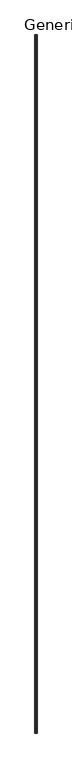
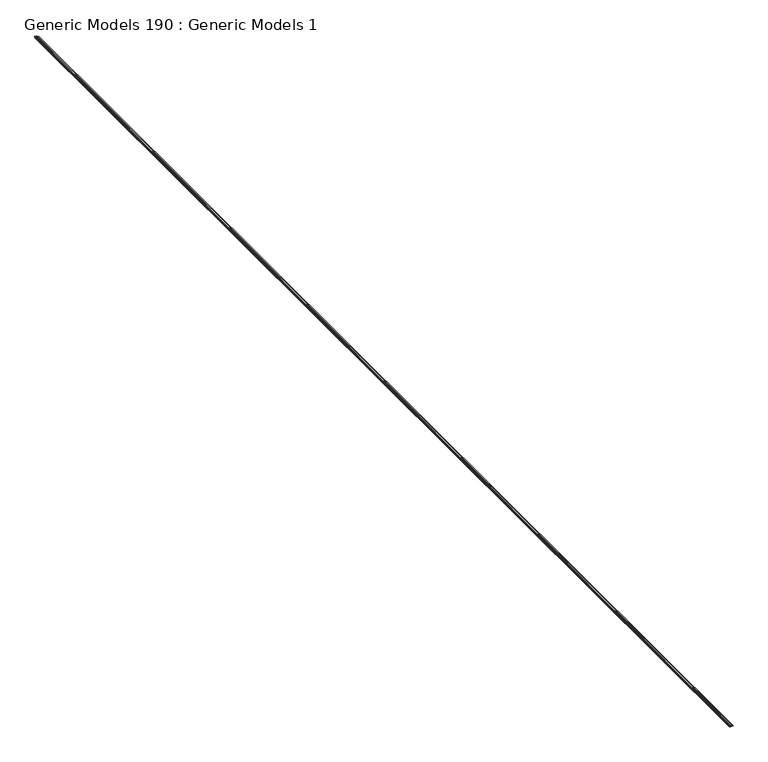
"""IFC4 building model written with IfcOpenShell, lengths in millimetres: proxy geometry, Generic Models 190 : Generic Models 1."""

from ifc_helpers import new_model, si_unit, frame, origin, place, context, project, spatial, polyline, outline, extrude, source, transform, mapped, element, save


def generic_models_190_generic_models_1_2642ba55(model_context):
    return source(origin(), model_context, "Body", "SweptSolid", [
        extrude(outline(polyline([(142599.5579199, -6986.3995748), (142601.7677199, -6986.3995748), (142601.7677199, -6985.5407339), (142622.0822986, -6985.5407339), (142622.0822986, -6986.8107339), (142603.0377199, -6986.8107339), (142603.0377199, -6987.6695748), (142598.2879199, -6987.6695748), (142598.2879199, -6965.4445748), (142609.7179199, -6965.4445748), (142609.7179199, -6952.7445748), (142598.2879199, -6952.7445748), (142598.2879199, -6929.0313908), (142599.5579199, -6929.0313908), (142599.5579199, -6951.4745748), (142610.9879199, -6951.4745748), (142610.9879199, -6966.7145748), (142599.5579199, -6966.7145748), (142599.5579199, -6986.3995748)])), frame((0.0, -7068.1230338, 0.0), z_axis=(0.0, 1.0, 0.0), x_axis=(0.0, 0.0, 1.0)), (0.0, 0.0, 1.0), 19050.0),
    ])


if __name__ == "__main__":
    model = new_model("IFC4")
    model_context = context("Model", 3, world=origin())
    ifc_project = project(units=[si_unit("LENGTHUNIT", "METRE", prefix="MILLI")], contexts=[model_context])
    site = spatial("IfcSite", under=ifc_project)
    building = spatial("IfcBuilding", under=site)
    placement = place(None, origin())
    generic_models_190_generic_models_1_shape = generic_models_190_generic_models_1_2642ba55(model_context)
    element("IfcBuildingElementProxy", 1, Name="Generic Models 190 : Generic Models 1", ObjectType="Generic Models 190 : Generic Models 1", at=placement, inside=building, context=model_context, shape_type="MappedRepresentation", body=[
        mapped(generic_models_190_generic_models_1_shape, transform((0.0, 0.0, 0.0), x_axis=(1.0, 0.0, 0.0), y_axis=(0.0, 1.0, 0.0), z_axis=(0.0, 0.0, 1.0))),
    ])
    save(model, "model.ifc")

# Revit data of these elements
# Element 1 (IfcBuildingElementProxy, "Generic Models 190 : Generic Models 1")
#   Materials on its faces: "_16 GA. COPPER SOFFIT DRIP SCREED"
# Materials
#   "_16 GA. COPPER SOFFIT DRIP SCREED": class "Generic", colour RGB 253 192 103, transparency 0, Cost = 0
